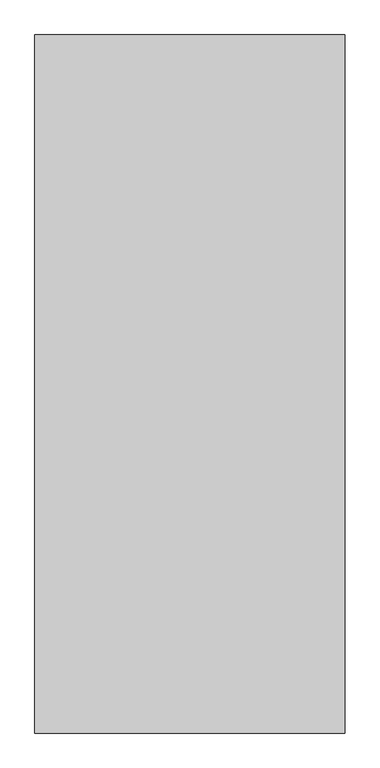
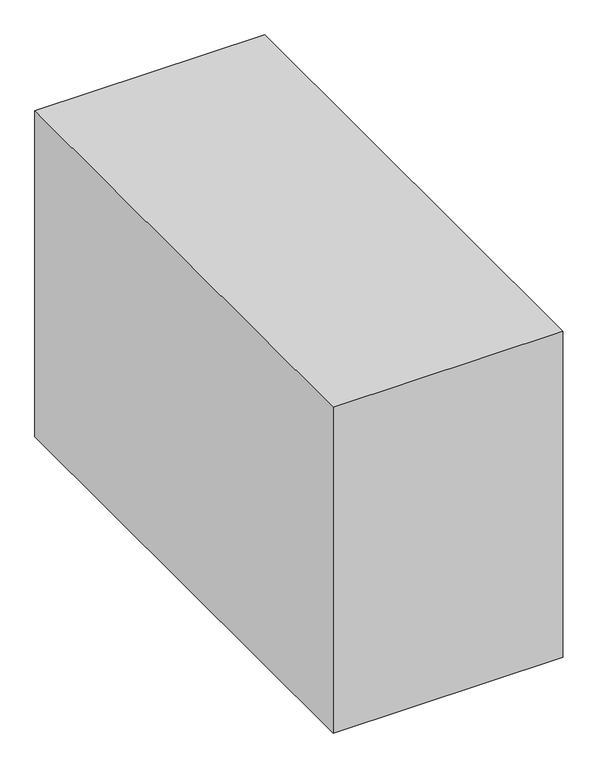
"""IFC4 building model written with IfcOpenShell, lengths in millimetres: proxy geometry, Space Planning Box_hec : Space Planning Box_hec."""

import ifcopenshell
import ifcopenshell.guid

model = None  # the IFC model being written
_history = None  # IfcOwnerHistory: only IFC2X3 demands one
_inside = {}  # id of a spatial element -> (the spatial element, [elements in it])
_under = {}  # id of a project, library or spatial element -> (it, [spatial elements below it])
_declared = {}  # id of a project -> (the project, [libraries it declares])
_typed = {}  # id of a type object -> (the type object, [elements of that type])
_made_of = {}  # id of a material, layer set ... -> (it, [elements and type objects made of it])


def new_model(schema):
    """Start an empty IFC model of exactly this schema.

    Asked for "IFC4X3", IfcOpenShell would pick the latest addendum, in which some entities
    have other attributes; the version numbers below select the first issue.
    IFC2X3 requires an IfcOwnerHistory on every rooted entity: one is made here for all.
    """
    global model, _history
    if schema == "IFC4X3":
        model = ifcopenshell.file(schema_version=(4, 3, 0, 0))
    else:
        model = ifcopenshell.file(schema=schema)
    _inside.clear()
    _under.clear()
    _declared.clear()
    _typed.clear()
    _made_of.clear()
    _history = None
    if model.schema == "IFC2X3":
        org = make("IfcOrganization", Name="unknown")
        user = make(
            "IfcPersonAndOrganization",
            ThePerson=make("IfcPerson", FamilyName="unknown"),
            TheOrganization=org,
        )
        app = make(
            "IfcApplication",
            ApplicationDeveloper=org,
            Version="unknown",
            ApplicationFullName="unknown",
            ApplicationIdentifier="unknown",
        )
        _history = make(
            "IfcOwnerHistory",
            OwningUser=user,
            OwningApplication=app,
            ChangeAction="ADDED",
            CreationDate=0,
        )
    return model


def make(cls, **values):
    """One entity of the class cls with the attributes given. An attribute that is None is left unset."""
    return model.create_entity(
        cls, **{name: value for name, value in values.items() if value is not None}
    )


def rooted(cls, **values):
    """An entity with a GlobalId (a new one), such as an element, a storey or a relation."""
    return make(cls, GlobalId=ifcopenshell.guid.new(), OwnerHistory=_history, **values)


def si_unit(unit_type, name, prefix=None):
    """IfcSIUnit, for example si_unit("LENGTHUNIT", "METRE", prefix="MILLI")."""
    return make("IfcSIUnit", UnitType=unit_type, Prefix=prefix, Name=name)


def assignment(units):
    """IfcUnitAssignment: the units of a project."""
    return None if units is None else make("IfcUnitAssignment", Units=units)


def point(xyz):
    """IfcCartesianPoint."""
    return None if xyz is None else make("IfcCartesianPoint", Coordinates=xyz)


def direction(xyz):
    """IfcDirection."""
    return None if xyz is None else make("IfcDirection", DirectionRatios=xyz)


def frame(location, z_axis=None, x_axis=None):
    """IfcAxis2Placement3D, a coordinate frame: its origin and axes. An axis left out is left unset."""
    return make(
        "IfcAxis2Placement3D",
        Location=point(location),
        Axis=direction(z_axis),
        RefDirection=direction(x_axis),
    )


def origin():
    """The frame at (0, 0, 0) with its axes left unset."""
    return frame((0.0, 0.0, 0.0))


def origin_with_axes():
    """The frame at (0, 0, 0) with the z axis (0, 0, 1) and the x axis (1, 0, 0) written out."""
    return frame((0.0, 0.0, 0.0), z_axis=(0.0, 0.0, 1.0), x_axis=(1.0, 0.0, 0.0))


def place(relative_to, where):
    """IfcLocalPlacement: puts the frame where relative to a parent placement (None: the world)."""
    return make(
        "IfcLocalPlacement", PlacementRelTo=relative_to, RelativePlacement=where
    )


def context(
    kind, dimensions, precision=None, world=None, true_north=None, identifier=None
):
    """IfcGeometricRepresentationContext, for example the 3D "Model" context."""
    return make(
        "IfcGeometricRepresentationContext",
        ContextIdentifier=identifier,
        ContextType=kind,
        CoordinateSpaceDimension=dimensions,
        Precision=precision,
        WorldCoordinateSystem=world,
        TrueNorth=true_north,
    )


def project(units=None, contexts=None):
    """IfcProject with its units and contexts."""
    return rooted(
        "IfcProject",
        Name="project",
        RepresentationContexts=contexts,
        UnitsInContext=assignment(units),
    )


def spatial(cls, under=None, at=None, **own):
    """A site, building, storey or space (cls), placed at a placement, below another one or the project."""
    s = rooted(cls, ObjectPlacement=at, **own)
    if under is not None:
        _under.setdefault(under.id(), (under, []))[1].append(s)
    return s


def polyline(points):
    """IfcPolyline through the points."""
    return make("IfcPolyline", Points=[point(p) for p in points])


def outline(outer, holes=None, kind="AREA"):
    """IfcArbitraryClosedProfileDef: a profile drawn as a closed curve; with holes, ...WithVoids."""
    if holes is None:
        return make("IfcArbitraryClosedProfileDef", ProfileType=kind, OuterCurve=outer)
    return make(
        "IfcArbitraryProfileDefWithVoids",
        ProfileType=kind,
        OuterCurve=outer,
        InnerCurves=holes,
    )


def extrude(swept, where, along, depth):
    """IfcExtrudedAreaSolid: the profile swept, set in the frame where, extruded along a direction by depth."""
    return make(
        "IfcExtrudedAreaSolid",
        SweptArea=swept,
        Position=where,
        ExtrudedDirection=direction(along),
        Depth=depth,
    )


def shape(context_of_items, identifier, shape_type, items):
    """IfcShapeRepresentation: the items that make up one representation, for example the "Body"."""
    return make(
        "IfcShapeRepresentation",
        ContextOfItems=context_of_items,
        RepresentationIdentifier=identifier,
        RepresentationType=shape_type,
        Items=items,
    )


def source(mapping_origin, context_of_items, identifier, shape_type, items):
    """IfcRepresentationMap: a shape defined once, which mapped items show again and again."""
    return make(
        "IfcRepresentationMap",
        MappingOrigin=mapping_origin,
        MappedRepresentation=shape(context_of_items, identifier, shape_type, items),
    )


def transform(
    local_origin,
    x_axis=None,
    y_axis=None,
    z_axis=None,
    scale=None,
    scale2=None,
    scale3=None,
    uniform=True,
):
    """IfcCartesianTransformationOperator3D, or its non-uniform kind. x_axis, y_axis, z_axis: its Axis1, 2, 3."""
    if uniform:
        return make(
            "IfcCartesianTransformationOperator3D",
            Axis1=direction(x_axis),
            Axis2=direction(y_axis),
            LocalOrigin=point(local_origin),
            Scale=scale,
            Axis3=direction(z_axis),
        )
    return make(
        "IfcCartesianTransformationOperator3DnonUniform",
        Axis1=direction(x_axis),
        Axis2=direction(y_axis),
        LocalOrigin=point(local_origin),
        Scale=scale,
        Axis3=direction(z_axis),
        Scale2=scale2,
        Scale3=scale3,
    )


def mapped(mapping_source, mapping_target):
    """IfcMappedItem: shows the shape of a source again, moved by a transform."""
    return make(
        "IfcMappedItem", MappingSource=mapping_source, MappingTarget=mapping_target
    )


def made_of(thing, what):
    """Note that an element or type object is made of a material, layer set ...; save() writes the relation."""
    if what is not None:
        _made_of.setdefault(what.id(), (what, []))[1].append(thing)
    return thing


def element(
    cls,
    number,
    at=None,
    inside=None,
    cuts=None,
    type_object=None,
    material=None,
    context=None,
    identifier="Body",
    shape_type=None,
    held_by="IfcProductDefinitionShape",
    body=None,
    shapes=None,
    **own,
):
    """One element of the class cls, such as IfcWall. Its Tag is "e" and its number.

    at: its placement. inside: the storey or other place that contains it. cuts: it is an
    opening in that element (IfcRelVoidsElement). A single representation is given by context,
    identifier, shape_type and body (its items); several are given by shapes. held_by: the class
    of the entity that holds the representations. save() writes the other relations.
    """
    e = rooted(cls, Tag="e%d" % number, ObjectPlacement=at, **own)
    if body is not None:
        shapes = [shape(context, identifier, shape_type, body)]
    if shapes is not None:
        e.Representation = make(held_by, Representations=shapes)
    if inside is not None:
        _inside.setdefault(inside.id(), (inside, []))[1].append(e)
    if cuts is not None:
        rooted(
            "IfcRelVoidsElement", RelatingBuildingElement=cuts, RelatedOpeningElement=e
        )
    if type_object is not None:
        _typed.setdefault(type_object.id(), (type_object, []))[1].append(e)
    return made_of(e, material)


def aggregate(whole, parts):
    """IfcRelAggregates: a whole, such as a stair, and the parts it consists of."""
    return rooted("IfcRelAggregates", RelatingObject=whole, RelatedObjects=parts)


def save(model, path):
    """Write the relations noted so far, then the file.

    IfcRelAggregates (storeys below a building ...), IfcRelContainedInSpatialStructure (elements
    in a storey), IfcRelDefinesByType, IfcRelAssociatesMaterial and IfcRelDeclares: one each for
    every whole, place, type object, material and project.
    """
    for whole, parts in _under.values():
        aggregate(whole, parts)
    for where, things in _inside.values():
        rooted(
            "IfcRelContainedInSpatialStructure",
            RelatedElements=things,
            RelatingStructure=where,
        )
    for kind, things in _typed.values():
        rooted("IfcRelDefinesByType", RelatedObjects=things, RelatingType=kind)
    for what, things in _made_of.values():
        rooted("IfcRelAssociatesMaterial", RelatedObjects=things, RelatingMaterial=what)
    for by, libraries in _declared.values():
        rooted("IfcRelDeclares", RelatingContext=by, RelatedDefinitions=libraries)
    model.write(path)


def generic_models_29bcd6f9(model_context):
    return source(origin(), model_context, "Body", "SweptSolid", [
        extrude(outline(polyline([(2000.0, 4500.0), (2000.0, -4500.0), (-2000.0, -4500.0), (-2000.0, 4500.0), (2000.0, 4500.0)])), origin_with_axes(), (0.0, 0.0, 1.0), 6000.0),
    ])


if __name__ == "__main__":
    model = new_model("IFC4")
    model_context = context("Model", 3, world=origin())
    ifc_project = project(units=[si_unit("LENGTHUNIT", "METRE", prefix="MILLI")], contexts=[model_context])
    site = spatial("IfcSite", under=ifc_project)
    building = spatial("IfcBuilding", under=site)
    placement = place(None, origin())
    generic_models_shape = generic_models_29bcd6f9(model_context)
    element("IfcBuildingElementProxy", 1, Name="Space Planning Box_hec : Space Planning Box_hec", ObjectType="Space Planning Box_hec : Space Planning Box_hec", at=placement, inside=building, context=model_context, shape_type="MappedRepresentation", body=[
        mapped(generic_models_shape, transform((0.0, 0.0, 0.0), x_axis=(1.0, 0.0, 0.0), y_axis=(0.0, 1.0, 0.0), z_axis=(0.0, 0.0, 1.0))),
    ])
    save(model, "model.ifc")

# Revit data of these elements
# Type "Space Planning Box_hec : Space Planning Box_hec"
#   Type Comments = "..."
#   Room Name [instance default] = "?"
#   Interior Finish [instance default] = ""
#   Exterior Finish [instance default] = ""
#   Department [instance default] = ""
#   Assembly Code = "..."
#   Width [instance default] = 1524 mm
#   Program Area [instance default] = 0.00 m²
#   Length [instance default] = 1524 mm
#   Height [instance default] = 1524 mm
#   Area [instance default] = 2.32258 m²
#   Fill Color [instance default] = Cyan
#   Default Elevation = 0
# Element 1 (IfcBuildingElementProxy, "Space Planning Box_hec : Space Planning Box_hec")
#   Room Name = "Stairway"
#   Interior Finish = "IF2"
#   Exterior Finish = "EF1"
#   Department = "AR"
#   Width = 4000 mm
#   Program Area = 36.00 m²
#   Length = 9000 mm
#   Height = 6000 mm
#   Area = 36.00 m²
#   Fill Color = Lavender
#   Materials on its faces: "Lavender"
# Materials
#   "Cyan": class "Generic", colour RGB 0 255 255, transparency 0.2, Cost = 0
#   "Lavender": class "Generic", colour RGB 186 85 211, transparency 0.2, Cost = 0
